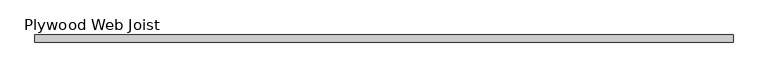
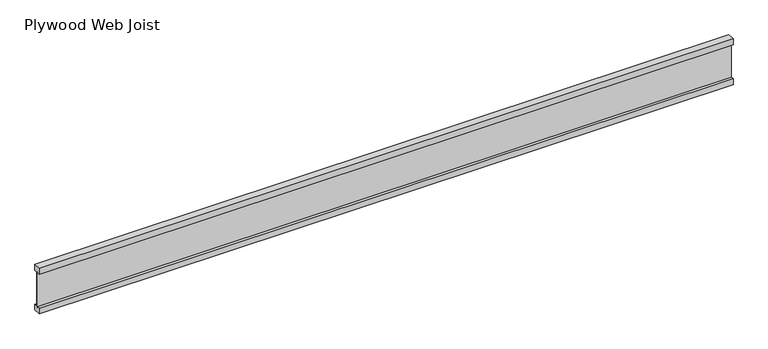
"""IFC4 building model written with IfcOpenShell, lengths in millimetres: beam geometry, Plywood Web Joist : TJI (T.B.D.)."""

from ifc_helpers import new_model, si_unit, frame, origin, place, context, project, spatial, polyline, outline, extrude, source, transform, mapped, element, save


def plywood_web_joist_98644929(model_context):
    return source(origin(), model_context, "Body", "SweptSolid", [
        extrude(outline(polyline([(-22.225, 150.8125), (22.225, 150.8125), (22.225, 112.7125), (4.7625, 112.7125), (4.7625, 119.0625), (-4.7625, 119.0625), (-4.7625, 112.7125), (-22.225, 112.7125), (-22.225, 150.8125)])), frame((-2163.9113281, 0.0, 0.0), z_axis=(1.0, 0.0, 0.0), x_axis=(0.0, 1.0, 0.0)), (0.0, 0.0, 1.0), 4337.1988281),
        extrude(outline(polyline([(22.225, -112.7125), (22.225, -150.8125), (-22.225, -150.8125), (-22.225, -112.7125), (-4.7625, -112.7125), (-4.7625, -118.3285374), (4.7625, -118.3285374), (4.7625, -112.7125), (22.225, -112.7125)])), frame((-2163.9113281, 0.0, 0.0), z_axis=(1.0, 0.0, 0.0), x_axis=(0.0, 1.0, 0.0)), (0.0, 0.0, 1.0), 4337.1988281),
        extrude(outline(polyline([(2173.2875, 4.7625), (2173.2875, -4.7625), (-2163.9113281, -4.7625), (-2163.9113281, 4.7625), (2173.2875, 4.7625)])), frame((0.0, 0.0, -118.3285374), z_axis=(0.0, 0.0, 1.0), x_axis=(1.0, 0.0, 0.0)), (0.0, 0.0, 1.0), 237.3910374),
    ])


if __name__ == "__main__":
    model = new_model("IFC4")
    model_context = context("Model", 3, world=origin())
    ifc_project = project(units=[si_unit("LENGTHUNIT", "METRE", prefix="MILLI")], contexts=[model_context])
    site = spatial("IfcSite", under=ifc_project)
    building = spatial("IfcBuilding", under=site)
    placement = place(None, origin())
    plywood_web_joist_shape = plywood_web_joist_98644929(model_context)
    element("IfcBeam", 1, ObjectType="Plywood Web Joist : TJI (T.B.D.)", at=placement, inside=building, context=model_context, shape_type="MappedRepresentation", body=[
        mapped(plywood_web_joist_shape, transform((0.0, 0.0, 0.0), x_axis=(1.0, 0.0, 0.0), y_axis=(0.0, 1.0, 0.0), z_axis=(0.0, 0.0, 1.0))),
    ])
    save(model, "model.ifc")

# Revit data of these elements
# Type "Plywood Web Joist : TJI (T.B.D.)"
#   Assembly Code = "B10"
#   Length [instance default] = 5' - 0"
#   b = 0' - 1 3/4"
#   d = 0' - 11 7/8"
#   Structural Material [instance default] = Softwood, Lumber
# Element 1 (IfcBeam, "Plywood Web Joist : TJI (T.B.D.)")
#   Materials on its faces: "Softwood, Lumber"
# Materials
#   "Softwood, Lumber": class "Wood", colour RGB 144 113 62, transparency 0, Description = "Pinus Echinata", Cost = 0
